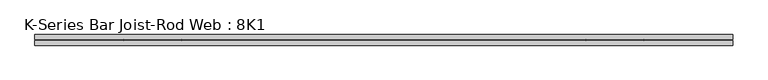
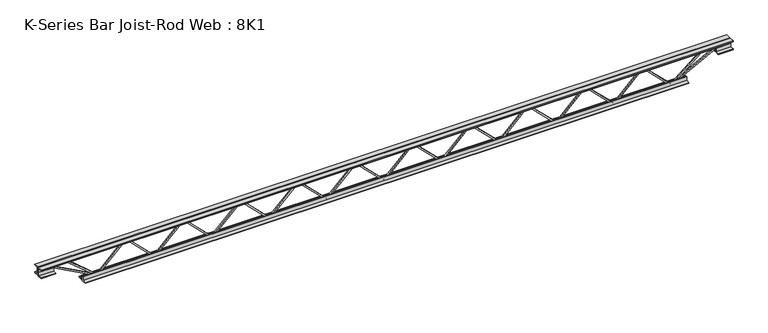
"""IFC4 building model written with IfcOpenShell, lengths in millimetres: beam geometry, K-Series Bar Joist-Rod Web : 8K1."""

from ifc_helpers import new_model, si_unit, frame, origin, place, context, project, spatial, polyline, outline, extrude, source, transform, mapped, element, save


def k_series_bar_joist_rod_web_8k1_7a100831(model_context):
    return source(origin(), model_context, "Body", "SweptSolid", [
        extrude(outline(polyline([(-90.4875, 1190.143393), (-100.0125, 1190.143393), (-100.0125, 1195.2801011), (90.4875, 1387.2873333), (90.4875, 1389.713917), (-100.0125, 1581.7211492), (-100.0125, 1586.8578573), (-90.4875, 1586.8578573), (-90.4875, 1585.6445655), (100.0125, 1393.6373333), (100.0125, 1383.363917), (-90.4875, 1191.3566849), (-90.4875, 1190.143393)])), frame((0.0, -4.7625, 0.0), z_axis=(0.0, 1.0, 0.0), x_axis=(0.0, 0.0, 1.0)), (0.0, 0.0, 1.0), 9.525),
        extrude(outline(polyline([(-90.4875, 793.4289287), (-100.0125, 793.4289287), (-100.0125, 798.5656368), (90.4875, 990.572869), (90.4875, 992.9994527), (-100.0125, 1185.0066849), (-100.0125, 1190.143393), (-90.4875, 1190.143393), (-90.4875, 1188.9301011), (100.0125, 996.922869), (100.0125, 986.6494527), (-90.4875, 794.6422205), (-90.4875, 793.4289287)])), frame((0.0, -4.7625, 0.0), z_axis=(0.0, 1.0, 0.0), x_axis=(0.0, 0.0, 1.0)), (0.0, 0.0, 1.0), 9.525),
        extrude(outline(polyline([(-90.4875, 396.7144643), (-100.0125, 396.7144643), (-100.0125, 401.8511725), (90.4875, 593.8584046), (90.4875, 596.2849884), (-100.0125, 788.2922205), (-100.0125, 793.4289287), (-90.4875, 793.4289287), (-90.4875, 792.2156368), (100.0125, 600.2084046), (100.0125, 589.9349884), (-90.4875, 397.9277562), (-90.4875, 396.7144643)])), frame((0.0, -4.7625, 0.0), z_axis=(0.0, 1.0, 0.0), x_axis=(0.0, 0.0, 1.0)), (0.0, 0.0, 1.0), 9.525),
        extrude(outline(polyline([(-90.4875, 0.0), (-100.0125, 0.0), (-100.0125, 5.1367081), (90.4875, 197.1439403), (90.4875, 199.570524), (-100.0125, 391.5777562), (-100.0125, 396.7144643), (-90.4875, 396.7144643), (-90.4875, 395.5011725), (100.0125, 203.4939403), (100.0125, 193.220524), (-90.4875, 1.2132919), (-90.4875, 0.0)])), frame((0.0, -4.7625, 0.0), z_axis=(0.0, 1.0, 0.0), x_axis=(0.0, 0.0, 1.0)), (0.0, 0.0, 1.0), 9.525),
        extrude(outline(polyline([(-90.4875, -396.7144643), (-100.0125, -396.7144643), (-100.0125, -391.5777562), (90.4875, -199.570524), (90.4875, -197.1439403), (-100.0125, -5.1367081), (-100.0125, 0.0), (-90.4875, 0.0), (-90.4875, -1.2132919), (100.0125, -193.220524), (100.0125, -203.4939403), (-90.4875, -395.5011725), (-90.4875, -396.7144643)])), frame((0.0, -4.7625, 0.0), z_axis=(0.0, 1.0, 0.0), x_axis=(0.0, 0.0, 1.0)), (0.0, 0.0, 1.0), 9.525),
        extrude(outline(polyline([(-90.4875, -793.4289287), (-100.0125, -793.4289287), (-100.0125, -788.2922205), (90.4875, -596.2849884), (90.4875, -593.8584046), (-100.0125, -401.8511725), (-100.0125, -396.7144643), (-90.4875, -396.7144643), (-90.4875, -397.9277562), (100.0125, -589.9349884), (100.0125, -600.2084046), (-90.4875, -792.2156368), (-90.4875, -793.4289287)])), frame((0.0, -4.7625, 0.0), z_axis=(0.0, 1.0, 0.0), x_axis=(0.0, 0.0, 1.0)), (0.0, 0.0, 1.0), 9.525),
        extrude(outline(polyline([(-90.4875, -1190.143393), (-100.0125, -1190.143393), (-100.0125, -1185.0066849), (90.4875, -992.9994527), (90.4875, -990.572869), (-100.0125, -798.5656368), (-100.0125, -793.4289287), (-90.4875, -793.4289287), (-90.4875, -794.6422205), (100.0125, -986.6494527), (100.0125, -996.922869), (-90.4875, -1188.9301011), (-90.4875, -1190.143393)])), frame((0.0, -4.7625, 0.0), z_axis=(0.0, 1.0, 0.0), x_axis=(0.0, 0.0, 1.0)), (0.0, 0.0, 1.0), 9.525),
        extrude(outline(polyline([(-90.4875, -1586.8578573), (-100.0125, -1586.8578573), (-100.0125, -1581.7211492), (90.4875, -1389.713917), (90.4875, -1387.2873333), (-100.0125, -1195.2801011), (-100.0125, -1190.143393), (-90.4875, -1190.143393), (-90.4875, -1191.3566849), (100.0125, -1383.363917), (100.0125, -1393.6373333), (-90.4875, -1585.6445655), (-90.4875, -1586.8578573)])), frame((0.0, -4.7625, 0.0), z_axis=(0.0, 1.0, 0.0), x_axis=(0.0, 0.0, 1.0)), (0.0, 0.0, 1.0), 9.525),
        extrude(outline(polyline([(-90.4875, 1586.8578573), (-100.0125, 1586.8578573), (-100.0125, 1591.9945655), (90.4875, 1784.0017976), (90.4875, 1786.4283814), (-100.0125, 1978.4356135), (-100.0125, 1983.5723217), (-90.4875, 1983.5723217), (-90.4875, 1982.3590298), (100.0125, 1790.3517976), (100.0125, 1780.0783814), (-90.4875, 1588.0711492), (-90.4875, 1586.8578573)])), frame((0.0, -4.7625, 0.0), z_axis=(0.0, 1.0, 0.0), x_axis=(0.0, 0.0, 1.0)), (0.0, 0.0, 1.0), 9.525),
        extrude(outline(polyline([(-90.4875, -1983.5723217), (-100.0125, -1983.5723217), (-100.0125, -1978.4356135), (90.4875, -1786.4283814), (90.4875, -1784.0017976), (-100.0125, -1591.9945655), (-100.0125, -1586.8578573), (-90.4875, -1586.8578573), (-90.4875, -1588.0711492), (100.0125, -1780.0783814), (100.0125, -1790.3517976), (-90.4875, -1982.3590298), (-90.4875, -1983.5723217)])), frame((0.0, -4.7625, 0.0), z_axis=(0.0, 1.0, 0.0), x_axis=(0.0, 0.0, 1.0)), (0.0, 0.0, 1.0), 9.525),
        extrude(outline(polyline([(4.7625, 101.6), (36.5125, 101.6), (36.5125, 95.25), (11.1125, 95.25), (11.1125, 69.85), (4.7625, 69.85), (4.7625, 101.6)])), frame((-2389.9723217, 0.0, 0.0), z_axis=(1.0, 0.0, 0.0), x_axis=(0.0, 1.0, 0.0)), (0.0, 0.0, 1.0), 4779.9446433),
        extrude(outline(polyline([(-4.7625, 101.6), (-4.7625, 69.85), (-11.1125, 69.85), (-11.1125, 95.25), (-36.5125, 95.25), (-36.5125, 101.6), (-4.7625, 101.6)])), frame((-2389.9723217, 0.0, 0.0), z_axis=(1.0, 0.0, 0.0), x_axis=(0.0, 1.0, 0.0)), (0.0, 0.0, 1.0), 4779.9446433),
        extrude(outline(polyline([(-4.7625, 38.1), (-36.5125, 38.1), (-36.5125, 44.45), (-11.1125, 44.45), (-11.1125, 69.85), (-4.7625, 69.85), (-4.7625, 38.1)])), frame((-2389.9723217, 0.0, 0.0), z_axis=(1.0, 0.0, 0.0), x_axis=(0.0, 1.0, 0.0)), (0.0, 0.0, 1.0), 101.6),
        extrude(outline(polyline([(36.5125, 38.1), (4.7625, 38.1), (4.7625, 69.85), (11.1125, 69.85), (11.1125, 44.45), (36.5125, 44.45), (36.5125, 38.1)])), frame((-2389.9723217, 0.0, 0.0), z_axis=(1.0, 0.0, 0.0), x_axis=(0.0, 1.0, 0.0)), (0.0, 0.0, 1.0), 101.6),
        extrude(outline(polyline([(4.7625, 38.1), (4.7625, 69.85), (11.1125, 69.85), (11.1125, 44.45), (36.5125, 44.45), (36.5125, 38.1), (4.7625, 38.1)])), frame((2288.3723217, 0.0, 0.0), z_axis=(1.0, 0.0, 0.0), x_axis=(0.0, 1.0, 0.0)), (0.0, 0.0, 1.0), 101.6),
        extrude(outline(polyline([(-4.7625, 38.1), (-36.5125, 38.1), (-36.5125, 44.45), (-11.1125, 44.45), (-11.1125, 69.85), (-4.7625, 69.85), (-4.7625, 38.1)])), frame((2288.3723217, 0.0, 0.0), z_axis=(1.0, 0.0, 0.0), x_axis=(0.0, 1.0, 0.0)), (0.0, 0.0, 1.0), 101.6),
        extrude(outline(polyline([(4.7625, -101.6), (4.7625, -69.85), (11.1125, -69.85), (11.1125, -95.25), (36.5125, -95.25), (36.5125, -101.6), (4.7625, -101.6)])), frame((-2085.1723217, 0.0, 0.0), z_axis=(1.0, 0.0, 0.0), x_axis=(0.0, 1.0, 0.0)), (0.0, 0.0, 1.0), 4170.3446433),
        extrude(outline(polyline([(-4.7625, -101.6), (-36.5125, -101.6), (-36.5125, -95.25), (-11.1125, -95.25), (-11.1125, -69.85), (-4.7625, -69.85), (-4.7625, -101.6)])), frame((-2085.1723217, 0.0, 0.0), z_axis=(1.0, 0.0, 0.0), x_axis=(0.0, 1.0, 0.0)), (0.0, 0.0, 1.0), 4170.3446433),
        extrude(outline(polyline([(0.0, -9.525), (0.0, 0.0), (346.6425392, 0.0), (346.6425392, -9.525), (0.0, -9.525)])), frame((-2290.6406201, 4.7625, 65.662372), z_axis=(0.47628314854008014, 0.0, 0.8792919665371384), x_axis=(0.8792919665371384, 0.0, -0.47628314854008014)), (0.0, 0.0, 1.0), 9.525),
        extrude(outline(polyline([(0.0, -9.525), (0.0, 0.0), (258.0767358, 0.0), (258.0767358, -9.525), (0.0, -9.525)])), frame((-2184.9762785, 4.7625, 66.1895526), z_axis=(0.6397322079385169, 0.0, 0.7685978806411778), x_axis=(0.7685978806411778, 0.0, -0.6397322079385169)), (0.0, 0.0, 1.0), 9.525),
        extrude(outline(polyline([(0.0, -9.525), (0.0, 0.0), (346.6425392, 0.0), (346.6425392, -9.525), (0.0, -9.525)])), frame((2290.6406201, -4.7625, 65.662372), z_axis=(-0.4762831485400428, 0.0, 0.8792919665371586), x_axis=(-0.8792919665371586, 0.0, -0.4762831485400428)), (0.0, 0.0, 1.0), 9.525),
        extrude(outline(polyline([(0.0, -9.525), (0.0, 0.0), (258.0767358, 0.0), (258.0767358, -9.525), (0.0, -9.525)])), frame((2184.9762785, -4.7625, 66.1895526), z_axis=(-0.6397322079384905, 0.0, 0.7685978806411997), x_axis=(-0.7685978806411997, 0.0, -0.6397322079384905)), (0.0, 0.0, 1.0), 9.525),
    ])


if __name__ == "__main__":
    model = new_model("IFC4")
    model_context = context("Model", 3, world=origin())
    ifc_project = project(units=[si_unit("LENGTHUNIT", "METRE", prefix="MILLI")], contexts=[model_context])
    site = spatial("IfcSite", under=ifc_project)
    building = spatial("IfcBuilding", under=site)
    placement = place(None, origin())
    k_series_bar_joist_rod_web_8k1_shape = k_series_bar_joist_rod_web_8k1_7a100831(model_context)
    element("IfcBeam", 1, ObjectType="K-Series Bar Joist-Rod Web : 8K1", at=placement, inside=building, context=model_context, shape_type="MappedRepresentation", body=[
        mapped(k_series_bar_joist_rod_web_8k1_shape, transform((0.0, 0.0, 0.0), x_axis=(1.0, 0.0, 0.0), y_axis=(0.0, 1.0, 0.0), z_axis=(0.0, 0.0, 1.0))),
    ])
    save(model, "model.ifc")

# Revit data of these elements
# Type "K-Series Bar Joist-Rod Web : 8K1"
#   Assembly Code = "B1010350"
#   Wt = 5.1
#   Web Thickness = 0' - 0 3/8"
#   Start Offset [instance default] = 0' - 0"
#   Start Extension [instance default] = 0' - 0"
#   Seat Length = 0' - 4"
#   Seat Depth = 0' - 2 1/2"
#   PanelArrayLength [instance default] = 21' - 4"
#   Panel [instance default] = 1' - 4"
#   End Offset [instance default] = 0' - 0"
#   End Extension [instance default] = 0' - 0"
#   End Panel = 1' - 4"
#   Cord Leg = 0' - 1 1/4"
#   Chord Thickness = 0' - 0 1/4"
#   Length [instance default] = 24' - 0"
#   Depth = 0' - 8"
#   PanelArrayNum [instance default] = 16
#   Rendering Material = none
# Element 1 (IfcBeam, "K-Series Bar Joist-Rod Web : 8K1")
#   PanelArrayLength = 13' - 0.1868"
#   Panel = 1' - 3.61868"
#   PanelArrayNum = 10
